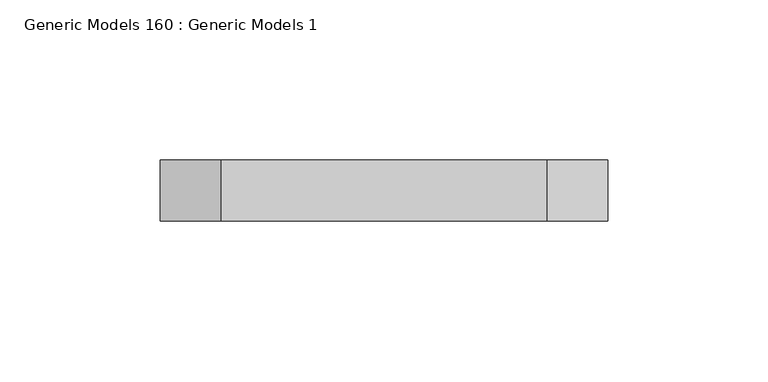
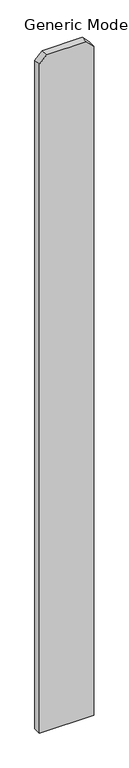
"""IFC4 building model written with IfcOpenShell, lengths in millimetres: proxy geometry, Generic Models 160 : Generic Models 1."""

from ifc_helpers import new_model, si_unit, frame, origin, place, context, project, spatial, polyline, outline, extrude, source, transform, mapped, element, save


def generic_models_160_generic_models_1_ee2fafda(model_context):
    return source(origin(), model_context, "Body", "SweptSolid", [
        extrude(outline(polyline([(76.2, -250420.1875), (1885.95, -250420.1875), (1905.0, -250439.2375), (1905.0, -250540.8375), (1885.95, -250559.8875), (76.2, -250559.8875), (76.2, -250420.1875)])), frame((0.0, 547.6875, 0.0), z_axis=(0.0, 1.0, 0.0), x_axis=(0.0, 0.0, 1.0)), (0.0, 0.0, 1.0), 19.05),
    ])


if __name__ == "__main__":
    model = new_model("IFC4")
    model_context = context("Model", 3, world=origin())
    ifc_project = project(units=[si_unit("LENGTHUNIT", "METRE", prefix="MILLI")], contexts=[model_context])
    site = spatial("IfcSite", under=ifc_project)
    building = spatial("IfcBuilding", under=site)
    placement = place(None, origin())
    generic_models_160_generic_models_1_shape = generic_models_160_generic_models_1_ee2fafda(model_context)
    element("IfcBuildingElementProxy", 1, Name="Generic Models 160 : Generic Models 1", ObjectType="Generic Models 160 : Generic Models 1", at=placement, inside=building, context=model_context, shape_type="MappedRepresentation", body=[
        mapped(generic_models_160_generic_models_1_shape, transform((0.0, 0.0, 0.0), x_axis=(1.0, 0.0, 0.0), y_axis=(0.0, 1.0, 0.0), z_axis=(0.0, 0.0, 1.0))),
    ])
    save(model, "model.ifc")

# Revit data of these elements
# Element 1 (IfcBuildingElementProxy, "Generic Models 160 : Generic Models 1")
#   Materials on its faces: "VERTICAL 1X6 CEDAR PLANKS W/ CLEAR WOOD SEALER"
# Materials
#   "VERTICAL 1X6 CEDAR PLANKS W/ CLEAR WOOD SEALER": class "Wood", colour RGB 234 198 147, transparency 0, Description = "Pinus Echinata", Cost = 0
